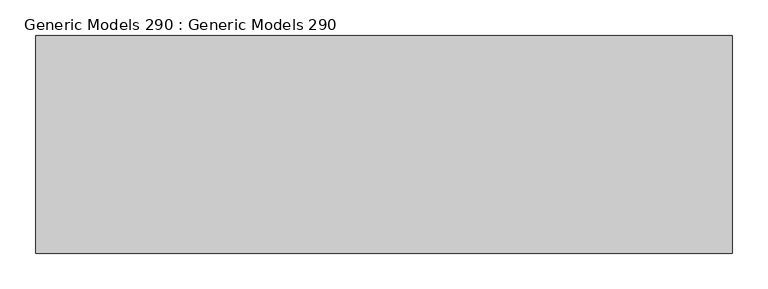
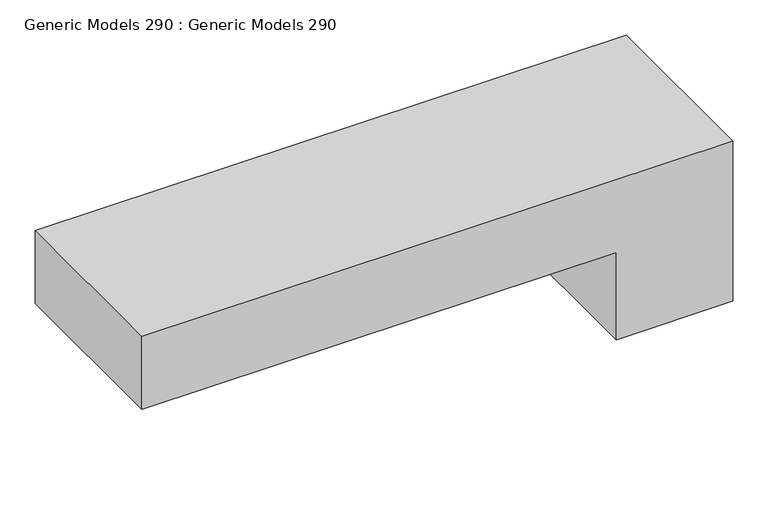
"""IFC4 building model written with IfcOpenShell, lengths in millimetres: proxy geometry, Generic Models 290 : Generic Models 290."""

import ifcopenshell
import ifcopenshell.guid

model = None  # the IFC model being written
_history = None  # IfcOwnerHistory: only IFC2X3 demands one
_inside = {}  # id of a spatial element -> (the spatial element, [elements in it])
_under = {}  # id of a project, library or spatial element -> (it, [spatial elements below it])
_declared = {}  # id of a project -> (the project, [libraries it declares])
_typed = {}  # id of a type object -> (the type object, [elements of that type])
_made_of = {}  # id of a material, layer set ... -> (it, [elements and type objects made of it])


def new_model(schema):
    """Start an empty IFC model of exactly this schema.

    Asked for "IFC4X3", IfcOpenShell would pick the latest addendum, in which some entities
    have other attributes; the version numbers below select the first issue.
    IFC2X3 requires an IfcOwnerHistory on every rooted entity: one is made here for all.
    """
    global model, _history
    if schema == "IFC4X3":
        model = ifcopenshell.file(schema_version=(4, 3, 0, 0))
    else:
        model = ifcopenshell.file(schema=schema)
    _inside.clear()
    _under.clear()
    _declared.clear()
    _typed.clear()
    _made_of.clear()
    _history = None
    if model.schema == "IFC2X3":
        org = make("IfcOrganization", Name="unknown")
        user = make(
            "IfcPersonAndOrganization",
            ThePerson=make("IfcPerson", FamilyName="unknown"),
            TheOrganization=org,
        )
        app = make(
            "IfcApplication",
            ApplicationDeveloper=org,
            Version="unknown",
            ApplicationFullName="unknown",
            ApplicationIdentifier="unknown",
        )
        _history = make(
            "IfcOwnerHistory",
            OwningUser=user,
            OwningApplication=app,
            ChangeAction="ADDED",
            CreationDate=0,
        )
    return model


def make(cls, **values):
    """One entity of the class cls with the attributes given. An attribute that is None is left unset."""
    return model.create_entity(
        cls, **{name: value for name, value in values.items() if value is not None}
    )


def rooted(cls, **values):
    """An entity with a GlobalId (a new one), such as an element, a storey or a relation."""
    return make(cls, GlobalId=ifcopenshell.guid.new(), OwnerHistory=_history, **values)


def si_unit(unit_type, name, prefix=None):
    """IfcSIUnit, for example si_unit("LENGTHUNIT", "METRE", prefix="MILLI")."""
    return make("IfcSIUnit", UnitType=unit_type, Prefix=prefix, Name=name)


def assignment(units):
    """IfcUnitAssignment: the units of a project."""
    return None if units is None else make("IfcUnitAssignment", Units=units)


def point(xyz):
    """IfcCartesianPoint."""
    return None if xyz is None else make("IfcCartesianPoint", Coordinates=xyz)


def direction(xyz):
    """IfcDirection."""
    return None if xyz is None else make("IfcDirection", DirectionRatios=xyz)


def frame(location, z_axis=None, x_axis=None):
    """IfcAxis2Placement3D, a coordinate frame: its origin and axes. An axis left out is left unset."""
    return make(
        "IfcAxis2Placement3D",
        Location=point(location),
        Axis=direction(z_axis),
        RefDirection=direction(x_axis),
    )


def origin():
    """The frame at (0, 0, 0) with its axes left unset."""
    return frame((0.0, 0.0, 0.0))


def place(relative_to, where):
    """IfcLocalPlacement: puts the frame where relative to a parent placement (None: the world)."""
    return make(
        "IfcLocalPlacement", PlacementRelTo=relative_to, RelativePlacement=where
    )


def context(
    kind, dimensions, precision=None, world=None, true_north=None, identifier=None
):
    """IfcGeometricRepresentationContext, for example the 3D "Model" context."""
    return make(
        "IfcGeometricRepresentationContext",
        ContextIdentifier=identifier,
        ContextType=kind,
        CoordinateSpaceDimension=dimensions,
        Precision=precision,
        WorldCoordinateSystem=world,
        TrueNorth=true_north,
    )


def project(units=None, contexts=None):
    """IfcProject with its units and contexts."""
    return rooted(
        "IfcProject",
        Name="project",
        RepresentationContexts=contexts,
        UnitsInContext=assignment(units),
    )


def spatial(cls, under=None, at=None, **own):
    """A site, building, storey or space (cls), placed at a placement, below another one or the project."""
    s = rooted(cls, ObjectPlacement=at, **own)
    if under is not None:
        _under.setdefault(under.id(), (under, []))[1].append(s)
    return s


def polyline(points):
    """IfcPolyline through the points."""
    return make("IfcPolyline", Points=[point(p) for p in points])


def outline(outer, holes=None, kind="AREA"):
    """IfcArbitraryClosedProfileDef: a profile drawn as a closed curve; with holes, ...WithVoids."""
    if holes is None:
        return make("IfcArbitraryClosedProfileDef", ProfileType=kind, OuterCurve=outer)
    return make(
        "IfcArbitraryProfileDefWithVoids",
        ProfileType=kind,
        OuterCurve=outer,
        InnerCurves=holes,
    )


def extrude(swept, where, along, depth):
    """IfcExtrudedAreaSolid: the profile swept, set in the frame where, extruded along a direction by depth."""
    return make(
        "IfcExtrudedAreaSolid",
        SweptArea=swept,
        Position=where,
        ExtrudedDirection=direction(along),
        Depth=depth,
    )


def shape(context_of_items, identifier, shape_type, items):
    """IfcShapeRepresentation: the items that make up one representation, for example the "Body"."""
    return make(
        "IfcShapeRepresentation",
        ContextOfItems=context_of_items,
        RepresentationIdentifier=identifier,
        RepresentationType=shape_type,
        Items=items,
    )


def source(mapping_origin, context_of_items, identifier, shape_type, items):
    """IfcRepresentationMap: a shape defined once, which mapped items show again and again."""
    return make(
        "IfcRepresentationMap",
        MappingOrigin=mapping_origin,
        MappedRepresentation=shape(context_of_items, identifier, shape_type, items),
    )


def transform(
    local_origin,
    x_axis=None,
    y_axis=None,
    z_axis=None,
    scale=None,
    scale2=None,
    scale3=None,
    uniform=True,
):
    """IfcCartesianTransformationOperator3D, or its non-uniform kind. x_axis, y_axis, z_axis: its Axis1, 2, 3."""
    if uniform:
        return make(
            "IfcCartesianTransformationOperator3D",
            Axis1=direction(x_axis),
            Axis2=direction(y_axis),
            LocalOrigin=point(local_origin),
            Scale=scale,
            Axis3=direction(z_axis),
        )
    return make(
        "IfcCartesianTransformationOperator3DnonUniform",
        Axis1=direction(x_axis),
        Axis2=direction(y_axis),
        LocalOrigin=point(local_origin),
        Scale=scale,
        Axis3=direction(z_axis),
        Scale2=scale2,
        Scale3=scale3,
    )


def mapped(mapping_source, mapping_target):
    """IfcMappedItem: shows the shape of a source again, moved by a transform."""
    return make(
        "IfcMappedItem", MappingSource=mapping_source, MappingTarget=mapping_target
    )


def made_of(thing, what):
    """Note that an element or type object is made of a material, layer set ...; save() writes the relation."""
    if what is not None:
        _made_of.setdefault(what.id(), (what, []))[1].append(thing)
    return thing


def element(
    cls,
    number,
    at=None,
    inside=None,
    cuts=None,
    type_object=None,
    material=None,
    context=None,
    identifier="Body",
    shape_type=None,
    held_by="IfcProductDefinitionShape",
    body=None,
    shapes=None,
    **own,
):
    """One element of the class cls, such as IfcWall. Its Tag is "e" and its number.

    at: its placement. inside: the storey or other place that contains it. cuts: it is an
    opening in that element (IfcRelVoidsElement). A single representation is given by context,
    identifier, shape_type and body (its items); several are given by shapes. held_by: the class
    of the entity that holds the representations. save() writes the other relations.
    """
    e = rooted(cls, Tag="e%d" % number, ObjectPlacement=at, **own)
    if body is not None:
        shapes = [shape(context, identifier, shape_type, body)]
    if shapes is not None:
        e.Representation = make(held_by, Representations=shapes)
    if inside is not None:
        _inside.setdefault(inside.id(), (inside, []))[1].append(e)
    if cuts is not None:
        rooted(
            "IfcRelVoidsElement", RelatingBuildingElement=cuts, RelatedOpeningElement=e
        )
    if type_object is not None:
        _typed.setdefault(type_object.id(), (type_object, []))[1].append(e)
    return made_of(e, material)


def aggregate(whole, parts):
    """IfcRelAggregates: a whole, such as a stair, and the parts it consists of."""
    return rooted("IfcRelAggregates", RelatingObject=whole, RelatedObjects=parts)


def save(model, path):
    """Write the relations noted so far, then the file.

    IfcRelAggregates (storeys below a building ...), IfcRelContainedInSpatialStructure (elements
    in a storey), IfcRelDefinesByType, IfcRelAssociatesMaterial and IfcRelDeclares: one each for
    every whole, place, type object, material and project.
    """
    for whole, parts in _under.values():
        aggregate(whole, parts)
    for where, things in _inside.values():
        rooted(
            "IfcRelContainedInSpatialStructure",
            RelatedElements=things,
            RelatingStructure=where,
        )
    for kind, things in _typed.values():
        rooted("IfcRelDefinesByType", RelatedObjects=things, RelatingType=kind)
    for what, things in _made_of.values():
        rooted("IfcRelAssociatesMaterial", RelatedObjects=things, RelatingMaterial=what)
    for by, libraries in _declared.values():
        rooted("IfcRelDeclares", RelatingContext=by, RelatedDefinitions=libraries)
    model.write(path)


def generic_models_290_generic_models_290_619c3f1e(model_context):
    return source(origin(), model_context, "Body", "SweptSolid", [
        extrude(outline(polyline([(123424.696, 6870.5263704), (123424.696, 5895.6570929), (123297.696, 5895.6570929), (123297.696, 6677.9290104), (123145.296, 6677.9290104), (123145.296, 6870.5263704), (123424.696, 6870.5263704)])), frame((0.0, 8214.8672747, 0.0), z_axis=(0.0, 1.0, 0.0), x_axis=(0.0, 0.0, 1.0)), (0.0, 0.0, 1.0), 304.8),
    ])


if __name__ == "__main__":
    model = new_model("IFC4")
    model_context = context("Model", 3, world=origin())
    ifc_project = project(units=[si_unit("LENGTHUNIT", "METRE", prefix="MILLI")], contexts=[model_context])
    site = spatial("IfcSite", under=ifc_project)
    building = spatial("IfcBuilding", under=site)
    placement = place(None, origin())
    generic_models_290_generic_models_290_shape = generic_models_290_generic_models_290_619c3f1e(model_context)
    element("IfcBuildingElementProxy", 1, Name="Generic Models 290 : Generic Models 290", ObjectType="Generic Models 290 : Generic Models 290", at=placement, inside=building, context=model_context, shape_type="MappedRepresentation", body=[
        mapped(generic_models_290_generic_models_290_shape, transform((0.0, 0.0, 0.0), x_axis=(1.0, 0.0, 0.0), y_axis=(0.0, 1.0, 0.0), z_axis=(0.0, 0.0, 1.0))),
    ])
    save(model, "model.ifc")

# Revit data of these elements
# Element 1 (IfcBuildingElementProxy, "Generic Models 290 : Generic Models 290")
#   Materials on its faces: "_ 8\" CONCRETE SLAB W/ GRADE BEAM (SEE STRUCT. DWGS)"
# Materials
#   "_ 8\" CONCRETE SLAB W/ GRADE BEAM (SEE STRUCT. DWGS)": class "Generic", colour RGB 191 191 191, transparency 0, Cost = 0
